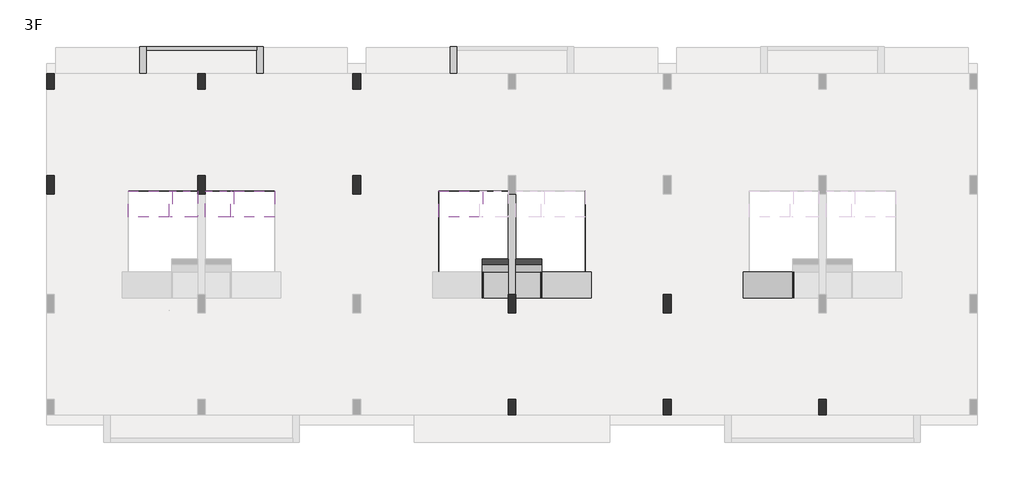
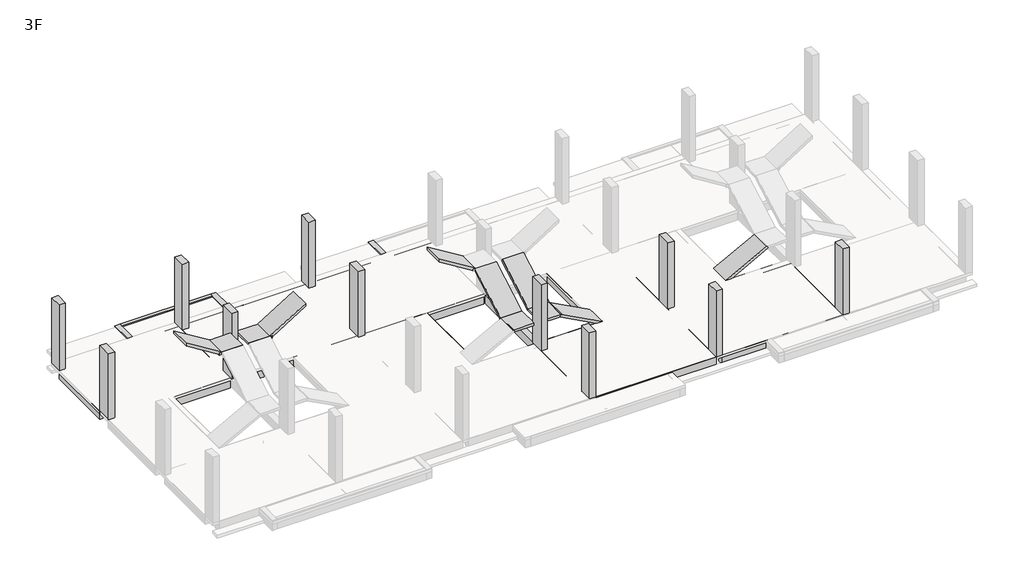
# One storey, part 2 of 3: 36 beams, 11 columns.
"""IFC4 building model written with IfcOpenShell, lengths in millimetres."""

from ifc_helpers import new_model, si_unit, frame, origin, place, context, project, spatial, polyline, outline, extrude, faceted_brep, element, save

model = new_model("IFC4")

# Units and contexts
model_context = context("Model", 3, world=origin())
ifc_project = project(units=[si_unit("LENGTHUNIT", "METRE", prefix="MILLI")], contexts=[model_context])

# Site, building, storey
site = spatial("IfcSite", under=ifc_project)
building = spatial("IfcBuilding", under=site)
storey = spatial("IfcBuildingStorey", under=building, Name="3F", Elevation=7330.0)

# Beams
placement = place(None, origin())
element("IfcBeam", 1, ObjectType="M_Concrete-Rectangular Beam : 1000x120", at=placement, inside=storey, context=model_context, shape_type="Brep", body=[
    faceted_brep([(4600.0000007, 7550.0000002, 9580.0), (4600.0000007, 8550.0000002, 9580.0), (4600.0000007, 8550.0000002, 9460.0), (4600.0000007, 7550.0000002, 9460.0), (5700.0000007, 8550.0000002, 9460.0), (5700.0000007, 8550.0000002, 9580.0), (5700.0000007, 7550.0000002, 9580.0), (5700.0000007, 7609.0063595, 9475.5095719), (5700.0000007, 7581.5414925, 9460.0), (4700.0000007, 7550.0000002, 9580.0), (4700.0000007, 7581.5414925, 9460.0), (4700.0000007, 7550.0000002, 9460.0), (4700.0000007, 7609.0063595, 9475.5095719)], [[[0, 1, 2, 3]], [[4, 5, 6, 7, 8]], [[1, 0, 9, 6, 5]], [[2, 1, 5, 4]], [[3, 2, 4, 8, 10, 11]], [[0, 3, 11, 9]], [[12, 7, 6, 9]], [[7, 12, 10, 8]], [[12, 9, 11, 10]]]),
])
element("IfcBeam", 2, ObjectType="M_Concrete-Rectangular Beam : 1000x120", at=placement, inside=storey, context=model_context, shape_type="Brep", body=[
    faceted_brep([(3019.99996, 7549.9999993, 10630.0), (4715.7503089, 7549.9999993, 9580.0), (4715.7503089, 8549.9999993, 9580.0), (3019.99996, 8549.9999993, 10630.0), (4600.0000007, 8549.9999993, 9580.0), (4600.0000007, 8549.9999993, 9510.5302519), (3020.0, 8549.9999993, 10488.8582245), (4600.0000007, 7549.9999993, 9510.5302519), (3020.0, 7549.9999993, 10488.8582245), (4600.0000007, 7549.9999993, 9580.0), (4700.0000007, 7549.9999993, 9580.0)], [[[0, 1, 2, 3]], [[3, 2, 4, 5, 6]], [[5, 7, 8, 6]], [[1, 0, 8, 7, 9, 10]], [[4, 9, 7, 5]], [[9, 4, 2, 1, 10]], [[0, 3, 6, 8]]]),
])
element("IfcBeam", 3, ObjectType="M_Concrete-Rectangular Beam : 1000x120", at=placement, inside=storey, context=model_context, shape_type="Brep", body=[
    faceted_brep([(7100.0000007, 8550.0000002, 9580.0), (7100.0000007, 7550.0000002, 9580.0), (7100.0000007, 7550.0000002, 9460.0), (7100.0000007, 8550.0000002, 9460.0), (6000.0000007, 8550.0000002, 9580.0), (6000.0000007, 8550.0000002, 9460.0), (6000.0000007, 7581.5414925, 9460.0), (6000.0000007, 7609.0063595, 9475.5095719), (6000.0000007, 7550.0000002, 9580.0), (7000.0000007, 7550.0000002, 9580.0), (7000.0000007, 7550.0000002, 9460.0), (7000.0000007, 7581.5414925, 9460.0), (7000.0000007, 7609.0063595, 9475.5095719)], [[[0, 1, 2, 3]], [[4, 5, 6, 7, 8]], [[1, 0, 4, 8, 9]], [[0, 3, 5, 4]], [[3, 2, 10, 11, 6, 5]], [[2, 1, 9, 10]], [[12, 9, 8, 7]], [[12, 7, 6, 11]], [[9, 12, 11, 10]]]),
])
element("IfcBeam", 4, ObjectType="M_Concrete-Rectangular Beam : 1000x120", at=placement, inside=storey, context=model_context, shape_type="Brep", body=[
    faceted_brep([(6984.2496926, 7549.9999993, 9580.0), (8680.0000414, 7549.9999993, 10630.0), (8680.0, 8549.9999993, 10629.9999744), (6984.2496926, 8549.9999993, 9580.0), (8680.0, 8549.9999993, 10488.8582236), (7100.0000007, 8549.9999993, 9510.5302519), (7100.0000007, 8549.9999993, 9580.0), (7100.0000007, 7549.9999993, 9510.5302519), (8680.0, 7549.9999993, 10488.8582236), (7000.0000007, 7549.9999993, 9580.0), (7100.0000007, 7549.9999993, 9580.0)], [[[0, 1, 2, 3]], [[3, 2, 4, 5, 6]], [[7, 5, 4, 8]], [[1, 0, 9, 10, 7, 8]], [[10, 6, 5, 7]], [[6, 10, 9, 0, 3]], [[2, 1, 8, 4]]]),
])
element("IfcBeam", 5, ObjectType="M_Concrete-Rectangular Beam : 1000x120", at=placement, inside=storey, context=model_context, shape_type="Brep", body=[
    faceted_brep([(16700.0000058, 7550.0000002, 9580.0), (17700.0000058, 7550.0000002, 9580.0), (17700.0000058, 7609.0063595, 9475.5095719), (16700.0000058, 7609.0063595, 9475.5095719), (16700.0000058, 5424.9999998, 8380.0), (16700.0000058, 5484.0063591, 8275.5095719), (17700.0000058, 5484.0063591, 8275.5095719), (17700.0000058, 5424.9999998, 8380.0), (17700.0000058, 5524.9999998, 8298.6589219), (17700.0000058, 7581.5414925, 9460.0), (16700.0000058, 5524.9999998, 8298.6589219), (16700.0000058, 7581.5414925, 9460.0)], [[[0, 1, 2, 3]], [[4, 5, 6, 7]], [[1, 0, 4, 7]], [[2, 1, 7, 6, 8, 9]], [[3, 2, 9, 8, 6, 5, 10, 11]], [[0, 3, 11, 10, 5, 4]]]),
])
element("IfcBeam", 6, ObjectType="M_Concrete-Rectangular Beam : 1000x120", at=placement, inside=storey, context=model_context, shape_type="Brep", body=[
    faceted_brep([(15019.9999651, 7549.9999993, 10630.0), (16715.7503139, 7549.9999993, 9580.0), (16715.7503139, 8549.9999993, 9580.0), (15019.9999651, 8549.9999993, 10630.0), (16600.0000058, 8549.9999993, 9580.0), (16600.0000058, 8549.9999993, 9510.5302519), (15020.0000057, 8549.9999993, 10488.8582241), (16600.0000058, 7549.9999993, 9510.5302519), (15020.0000057, 7549.9999993, 10488.8582241), (16600.0000058, 7549.9999993, 9580.0), (16700.0000058, 7549.9999993, 9580.0)], [[[0, 1, 2, 3]], [[3, 2, 4, 5, 6]], [[5, 7, 8, 6]], [[1, 0, 8, 7, 9, 10]], [[4, 9, 7, 5]], [[9, 4, 2, 1, 10]], [[0, 3, 6, 8]]]),
])
element("IfcBeam", 7, ObjectType="M_Concrete-Rectangular Beam : 1000x120", at=placement, inside=storey, context=model_context, shape_type="Brep", body=[
    faceted_brep([(17700.0000058, 5524.9999998, 8260.0), (16700.0000058, 5524.9999998, 8260.0), (16700.0000058, 5524.9999998, 8298.6589219), (17700.0000058, 5524.9999998, 8298.6589219), (17700.0000058, 4424.9999998, 8260.0), (17700.0000058, 4424.9999998, 8380.0), (16730.4772117, 4424.9999998, 8380.0), (16787.1330628, 4424.9999998, 8274.2166623), (16760.588832, 4424.9999998, 8260.0), (17700.0000058, 5424.9999998, 8380.0), (16700.0000058, 5424.9999998, 8380.0), (16700.0000058, 4424.9999998, 8380.0), (17700.0000058, 5484.0063591, 8275.5095719), (16760.588832, 5424.9999998, 8260.0), (16700.0000058, 5424.9999998, 8260.0), (16700.0000058, 4424.9999998, 8363.6768996), (16700.0000058, 5484.0063591, 8275.5095719), (16700.0000058, 5424.9999998, 8363.6768996), (16730.4772117, 5424.9999998, 8380.0), (16787.1330628, 5424.9999998, 8274.2166623)], [[[0, 1, 2, 3]], [[4, 5, 6, 7, 8]], [[6, 5, 9, 10, 11]], [[5, 4, 0, 3, 12, 9]], [[1, 0, 4, 8, 13, 14]], [[15, 11, 10, 16, 2, 1, 14, 17]], [[6, 18, 19, 7]], [[18, 6, 15, 17]], [[7, 19, 13, 8]], [[19, 18, 17, 14, 13]], [[11, 15, 6]], [[12, 16, 10, 9]], [[16, 12, 3, 2]]]),
])
element("IfcBeam", 8, ObjectType="M_Concrete-Rectangular Beam : 1000x120", at=placement, inside=storey, context=model_context, shape_type="Brep", body=[
    faceted_brep([(18969.5227998, 4424.9999998, 8380.0), (18969.5227998, 5424.9999998, 8380.0), (18912.8669488, 5424.9999998, 8274.2166623), (18912.8669488, 4424.9999998, 8274.2166623), (19000.0000058, 4424.9999998, 8363.6768996), (20930.0000065, 4424.9999998, 7330.0), (20930.0000065, 5424.9999998, 7330.0), (19000.0000058, 5424.9999998, 8363.6768996), (18939.4111796, 4424.9999998, 8260.0), (20675.8338483, 4424.9999998, 7330.0), (18939.4111796, 5424.9999998, 8260.0), (20680.0000058, 5424.9999998, 7327.7686732), (20680.0000058, 4449.9999998, 7327.7686732), (20675.8338483, 4449.9999998, 7330.0), (20680.0000058, 5424.9999998, 7330.0), (20680.0000058, 4449.9999998, 7330.0)], [[[0, 1, 2, 3]], [[1, 0, 4, 5, 6, 7]], [[0, 3, 8, 9, 5, 4]], [[3, 2, 10, 11, 12, 13, 9, 8]], [[2, 1, 7, 6, 14, 11, 10]], [[9, 13, 15, 14, 6, 5]], [[11, 14, 15, 12]], [[15, 13, 12]]]),
])
element("IfcBeam", 9, ObjectType="M_Concrete-Rectangular Beam : 1000x120", at=placement, inside=storey, context=model_context, shape_type="Brep", body=[
    faceted_brep([(19000.0000058, 7550.0000002, 9580.0), (19000.0000058, 7609.0063595, 9475.5095719), (18000.0000058, 7609.0063595, 9475.5095719), (18000.0000058, 7550.0000002, 9580.0), (19000.0000058, 5424.9999998, 8380.0), (18000.0000058, 5424.9999998, 8380.0), (18000.0000058, 5484.0063591, 8275.5095719), (19000.0000058, 5484.0063591, 8275.5095719), (18000.0000058, 7581.5414925, 9460.0), (18000.0000058, 5524.9999998, 8298.6589219), (19000.0000058, 7581.5414925, 9460.0), (19000.0000058, 5524.9999998, 8298.6589219)], [[[0, 1, 2, 3]], [[4, 5, 6, 7]], [[3, 5, 4, 0]], [[2, 8, 9, 6, 5, 3]], [[1, 10, 11, 7, 6, 9, 8, 2]], [[0, 4, 7, 11, 10, 1]]]),
])
element("IfcBeam", 10, ObjectType="M_Concrete-Rectangular Beam : 1000x120", at=placement, inside=storey, context=model_context, shape_type="Brep", body=[
    faceted_brep([(19000.0000058, 5524.9999998, 8260.0), (18000.0000058, 5524.9999998, 8260.0), (18000.0000058, 5524.9999998, 8298.6589219), (19000.0000058, 5524.9999998, 8298.6589219), (18000.0000058, 4424.9999998, 8380.0), (18000.0000058, 4424.9999998, 8260.0), (18939.4111796, 4424.9999998, 8260.0), (18912.8669488, 4424.9999998, 8274.2166623), (18969.5227998, 4424.9999998, 8380.0), (19000.0000058, 4424.9999998, 8380.0), (19000.0000058, 5424.9999998, 8380.0), (18000.0000058, 5424.9999998, 8380.0), (18000.0000058, 5484.0063591, 8275.5095719), (19000.0000058, 5424.9999998, 8260.0), (18939.4111796, 5424.9999998, 8260.0), (19000.0000058, 4424.9999998, 8363.6768996), (19000.0000058, 5424.9999998, 8363.6768996), (19000.0000058, 5484.0063591, 8275.5095719), (18969.5227998, 5424.9999998, 8380.0), (18912.8669488, 5424.9999998, 8274.2166623)], [[[0, 1, 2, 3]], [[4, 5, 6, 7, 8]], [[8, 9, 10, 11, 4]], [[5, 4, 11, 12, 2, 1]], [[1, 0, 13, 14, 6, 5]], [[9, 15, 16, 13, 0, 3, 17, 10]], [[18, 8, 7, 19]], [[8, 18, 16, 15]], [[19, 7, 6, 14]], [[18, 19, 14, 13, 16]], [[15, 9, 8]], [[17, 12, 11, 10]], [[12, 17, 3, 2]]]),
])
element("IfcBeam", 11, ObjectType="M_Concrete-Rectangular Beam : 1000x120", at=placement, inside=storey, context=model_context, shape_type="Brep", body=[
    faceted_brep([(28730.4772098, 5424.9999998, 8380.0), (28730.4772098, 4424.9999998, 8380.0), (28787.1330609, 4424.9999998, 8274.2166623), (28787.1330609, 5424.9999998, 8274.2166623), (28700.0000039, 5424.9999998, 8363.6768996), (26770.0000031, 5424.9999998, 7330.0), (26770.0000031, 4424.9999998, 7330.0), (28700.0000039, 4424.9999998, 8363.6768996), (27024.1661613, 4424.9999998, 7330.0), (28760.5888301, 4424.9999998, 8260.0), (27024.1661613, 4449.9999998, 7330.0), (27020.000004, 4449.9999998, 7327.7686733), (27020.000004, 5424.9999998, 7327.7686733), (28760.5888301, 5424.9999998, 8260.0), (27020.000004, 5424.9999998, 7330.0), (27020.000004, 4449.9999998, 7330.0)], [[[0, 1, 2, 3]], [[1, 0, 4, 5, 6, 7]], [[2, 1, 7, 6, 8, 9]], [[3, 2, 9, 8, 10, 11, 12, 13]], [[0, 3, 13, 12, 14, 5, 4]], [[5, 14, 15, 10, 8, 6]], [[14, 12, 11, 15]], [[10, 15, 11]]]),
])
element("IfcBeam", 12, ObjectType="M_Concrete-Rectangular Beam : 150x500", at=placement, inside=storey, context=model_context, shape_type="SweptSolid", body=[
    extrude(outline(polyline([(7990.0000277, 14150.0000066), (7990.0000277, 14000.0000066), (3709.9999747, 14000.0000066), (3709.9999747, 14150.0000066), (7990.0000277, 14150.0000066)])), frame((0.0, 0.0, 6830.0), z_axis=(0.0, 0.0, 1.0), x_axis=(1.0, 0.0, 0.0)), (0.0, 0.0, 1.0), 500.0),
])
element("IfcBeam", 13, ObjectType="M_Concrete-Rectangular Beam : 250x400", at=placement, inside=storey, context=model_context, shape_type="Brep", body=[
    faceted_brep([(20930.0000058, 8549.9999993, 7330.0), (20680.0000058, 8549.9999993, 7330.0), (20680.0000058, 5424.9999998, 7330.0), (20680.0000058, 4449.9999998, 7330.0), (20930.0000058, 4449.9999998, 7330.0), (20680.0000058, 8549.9999993, 7188.8582241), (20680.0000058, 8549.9999993, 6930.0), (20680.0000058, 4449.9999998, 6930.0), (20680.0000058, 4449.9999998, 7327.7686732), (20930.0000058, 8549.9999993, 6930.0), (20930.0000058, 4449.9999998, 6930.0)], [[[0, 1, 2, 3, 4]], [[1, 5, 6, 7, 8, 3, 2]], [[6, 9, 10, 7]], [[9, 0, 4, 10]], [[1, 0, 9, 6, 5]], [[4, 3, 8, 7, 10]]]),
])
element("IfcBeam", 14, ObjectType="M_Concrete-Rectangular Beam : 250x400", at=placement, inside=storey, context=model_context, shape_type="Brep", body=[
    faceted_brep([(15020.0000057, 8549.9999993, 7330.0), (14770.0000057, 8549.9999993, 7330.0), (14770.0000057, 4449.9999998, 7330.0), (15020.0000057, 4449.9999998, 7330.0), (15020.0000057, 5424.9999998, 7330.0), (15020.0000057, 8549.9999993, 6930.0), (15020.0000057, 8549.9999993, 7188.8582241), (15020.0000057, 4449.9999998, 7327.7686732), (15020.0000057, 4449.9999998, 6930.0), (14770.0000057, 8549.9999993, 6930.0), (14770.0000057, 4449.9999998, 6930.0)], [[[0, 1, 2, 3, 4]], [[5, 6, 0, 4, 3, 7, 8]], [[9, 5, 8, 10]], [[1, 9, 10, 2]], [[1, 0, 6, 5, 9]], [[3, 2, 10, 8, 7]]]),
])
element("IfcBeam", 15, ObjectType="M_Concrete-Rectangular Beam : 250x500", at=placement, inside=storey, context=model_context, shape_type="Brep", body=[
    faceted_brep([(8240.0000277, 14150.0000066, 7330.0), (7990.0000277, 14150.0000066, 7330.0), (7990.0000277, 14000.0000066, 7330.0), (7990.0000277, 13100.0000001, 7330.0), (8240.0000277, 13100.0000001, 7330.0), (7990.0000277, 14150.0000066, 6830.0), (7990.0000277, 14000.0000066, 6830.0), (7990.0000277, 13100.0000001, 6830.0), (8240.0000277, 14150.0000066, 6830.0), (8240.0000277, 13100.0000001, 6830.0)], [[[0, 1, 2, 3, 4]], [[1, 5, 6, 7, 3, 2]], [[5, 8, 9, 7, 6]], [[8, 0, 4, 9]], [[4, 3, 7, 9]], [[1, 0, 8, 5]]]),
])
element("IfcBeam", 16, ObjectType="M_Concrete-Rectangular Beam : 250x500", at=placement, inside=storey, context=model_context, shape_type="Brep", body=[
    faceted_brep([(3709.9999747, 14150.0000066, 7330.0), (3459.9999747, 14150.0000066, 7330.0), (3459.9999747, 13100.0000001, 7330.0), (3709.9999747, 13100.0000001, 7330.0), (3709.9999747, 14000.0000066, 7330.0), (3709.9999747, 14150.0000066, 6830.0), (3709.9999747, 13100.0000001, 6830.0), (3709.9999747, 14000.0000066, 6830.0), (3459.9999747, 14150.0000066, 6830.0), (3459.9999747, 13100.0000001, 6830.0)], [[[0, 1, 2, 3, 4]], [[5, 0, 4, 3, 6, 7]], [[8, 5, 7, 6, 9]], [[1, 8, 9, 2]], [[3, 2, 9, 6]], [[1, 0, 5, 8]]]),
])
element("IfcBeam", 17, ObjectType="M_Concrete-Rectangular Beam : 250x500", at=placement, inside=storey, context=model_context, shape_type="Brep", body=[
    faceted_brep([(15710.0998466, 14150.0000066, 7330.0), (15460.0998466, 14150.0000066, 7330.0), (15460.0998466, 13100.0000001, 7330.0), (15710.0998466, 13100.0000001, 7330.0), (15710.0998466, 14000.0000066, 7330.0), (15710.0998466, 14150.0000066, 6830.0), (15710.0998466, 13100.0000001, 6830.0), (15710.0998466, 14000.0000066, 6830.0), (15460.0998466, 14150.0000066, 6830.0), (15460.0998466, 13100.0000001, 6830.0)], [[[0, 1, 2, 3, 4]], [[5, 0, 4, 3, 6, 7]], [[8, 5, 7, 6, 9]], [[1, 8, 9, 2]], [[3, 2, 9, 6]], [[1, 0, 5, 8]]]),
])
element("IfcBeam", 18, ObjectType="M_Concrete-Rectangular Beam : 300x400", at=placement, inside=storey, context=model_context, shape_type="SweptSolid", body=[
    extrude(outline(polyline([(165.0, 9149.9985388), (-135.0, 9149.9985388), (-135.0, 12500.0000003), (165.0, 12500.0000003), (165.0, 9149.9985388)])), frame((0.0, 0.0, 6930.0), z_axis=(0.0, 0.0, 1.0), x_axis=(1.0, 0.0, 0.0)), (0.0, 0.0, 1.0), 400.0),
])
element("IfcBeam", 19, ObjectType="M_Concrete-Rectangular Beam : 300x400", at=placement, inside=storey, context=model_context, shape_type="SweptSolid", body=[
    extrude(outline(polyline([(18000.0000046, 4550.0000002), (17700.0000046, 4550.0000002), (17700.0000046, 8449.9985388), (18000.0000046, 8449.9985388), (18000.0000046, 4550.0000002)])), frame((0.0, 0.0, 6930.0), z_axis=(0.0, 0.0, 1.0), x_axis=(1.0, 0.0, 0.0)), (0.0, 0.0, 1.0), 400.0),
])
element("IfcBeam", 20, ObjectType="M_Concrete-Rectangular Beam : 300x400", at=placement, inside=storey, context=model_context, shape_type="SweptSolid", body=[
    extrude(outline(polyline([(18000.0000046, 499.9999998), (17700.0000046, 499.9999998), (17700.0000046, 3850.0000002), (18000.0000046, 3850.0000002), (18000.0000046, 499.9999998)])), frame((0.0, 0.0, 6930.0), z_axis=(0.0, 0.0, 1.0), x_axis=(1.0, 0.0, 0.0)), (0.0, 0.0, 1.0), 400.0),
])
element("IfcBeam", 21, ObjectType="M_Concrete-Rectangular Beam : 300x400", at=placement, inside=storey, context=model_context, shape_type="SweptSolid", body=[
    extrude(outline(polyline([(30000.0000031, 499.9999998), (29700.0000031, 499.9999998), (29700.0000031, 3850.0000002), (30000.0000031, 3850.0000002), (30000.0000031, 499.9999998)])), frame((0.0, 0.0, 6930.0), z_axis=(0.0, 0.0, 1.0), x_axis=(1.0, 0.0, 0.0)), (0.0, 0.0, 1.0), 400.0),
])
element("IfcBeam", 22, ObjectType="M_Concrete-Rectangular Beam : 300x400", at=placement, inside=storey, context=model_context, shape_type="SweptSolid", body=[
    extrude(outline(polyline([(24000.000004, 499.9999998), (23700.000004, 499.9999998), (23700.000004, 3850.0000002), (24000.000004, 3850.0000002), (24000.000004, 499.9999998)])), frame((0.0, 0.0, 6930.0), z_axis=(0.0, 0.0, 1.0), x_axis=(1.0, 0.0, 0.0)), (0.0, 0.0, 1.0), 400.0),
])
element("IfcBeam", 23, ObjectType="M_Concrete-Rectangular Beam : 300x400", at=placement, inside=storey, context=model_context, shape_type="SweptSolid", body=[
    extrude(outline(polyline([(24000.000004, 4550.0000002), (23700.000004, 4550.0000002), (23700.000004, 8449.9985388), (24000.000004, 8449.9985388), (24000.000004, 4550.0000002)])), frame((0.0, 0.0, 6930.0), z_axis=(0.0, 0.0, 1.0), x_axis=(1.0, 0.0, 0.0)), (0.0, 0.0, 1.0), 400.0),
])
element("IfcBeam", 24, ObjectType="M_Concrete-Rectangular Beam : 300x400", at=placement, inside=storey, context=model_context, shape_type="SweptSolid", body=[
    extrude(outline(polyline([(6000.0000007, 9149.9985388), (5700.0000007, 9149.9985388), (5700.0000007, 12500.0000003), (6000.0000007, 12500.0000003), (6000.0000007, 9149.9985388)])), frame((0.0, 0.0, 6930.0), z_axis=(0.0, 0.0, 1.0), x_axis=(1.0, 0.0, 0.0)), (0.0, 0.0, 1.0), 400.0),
])
element("IfcBeam", 25, ObjectType="M_Concrete-Rectangular Beam : 300x400", at=placement, inside=storey, context=model_context, shape_type="SweptSolid", body=[
    extrude(outline(polyline([(12000.0000034, 9149.9985388), (11700.0000034, 9149.9985388), (11700.0000034, 12500.0000003), (12000.0000034, 12500.0000003), (12000.0000034, 9149.9985388)])), frame((0.0, 0.0, 6930.0), z_axis=(0.0, 0.0, 1.0), x_axis=(1.0, 0.0, 0.0)), (0.0, 0.0, 1.0), 400.0),
])
element("IfcBeam", 26, ObjectType="M_Concrete-Rectangular Beam : 300x400", at=placement, inside=storey, context=model_context, shape_type="SweptSolid", body=[
    extrude(outline(polyline([(6000.0000007, 13100.0000003), (5700.0000007, 13100.0000001), (5700.0000007, 14000.0000066), (6000.0000007, 14000.0000066), (6000.0000007, 13100.0000003)])), frame((0.0, 0.0, 6880.0), z_axis=(0.0, 0.0, 1.0), x_axis=(1.0, 0.0, 0.0)), (0.0, 0.0, 1.0), 400.0),
])
element("IfcBeam", 27, ObjectType="M_Concrete-Rectangular Beam : 300x500", at=placement, inside=storey, context=model_context, shape_type="Brep", body=[
    faceted_brep([(164.9999993, 13100.0000001, 7330.0), (164.9999993, 12800.0000001, 7330.0), (5700.0000007, 12800.0000001, 7330.0), (5700.0000007, 13100.0000001, 7330.0), (3709.9999747, 13100.0000001, 7330.0), (3459.9999747, 13100.0000001, 7330.0), (164.9999993, 12800.0000001, 6830.0), (5700.0000007, 12800.0000001, 6830.0), (164.9999993, 13100.0000001, 6830.0), (3459.9999747, 13100.0000001, 6830.0), (3709.9999747, 13100.0000001, 6830.0), (5700.0000007, 13100.0000001, 6830.0)], [[[0, 1, 2, 3, 4, 5]], [[1, 6, 7, 2]], [[6, 8, 9, 10, 11, 7]], [[8, 0, 5, 4, 3, 11, 10, 9]], [[1, 0, 8, 6]], [[3, 2, 7, 11]]]),
])
element("IfcBeam", 28, ObjectType="M_Concrete-Rectangular Beam : 300x500", at=placement, inside=storey, context=model_context, shape_type="Brep", body=[
    faceted_brep([(165.0, 8849.9999993, 7330.0), (165.0, 8549.9999993, 7330.0), (2770.0, 8549.9999993, 7330.0), (3020.0, 8549.9999993, 7330.0), (5700.0000007, 8549.9999993, 7330.0), (5700.0000007, 8849.9999993, 7330.0), (165.0, 8549.9999993, 6830.0), (5700.0000007, 8549.9999993, 6830.0), (165.0, 8849.9999993, 6830.0), (5700.0000007, 8849.9999993, 6830.0)], [[[0, 1, 2, 3, 4, 5]], [[1, 6, 7, 4, 3, 2]], [[6, 8, 9, 7]], [[8, 0, 5, 9]], [[1, 0, 8, 6]], [[5, 4, 7, 9]]]),
])
element("IfcBeam", 29, ObjectType="M_Concrete-Rectangular Beam : 300x500", at=placement, inside=storey, context=model_context, shape_type="Brep", body=[
    faceted_brep([(6000.0000007, 13100.0000001, 7330.0), (6000.0000007, 12800.0000001, 7330.0), (11700.0000034, 12800.0000001, 7330.0), (11700.0000034, 13100.0000001, 7330.0), (8240.0000277, 13100.0000001, 7330.0), (7990.0000277, 13100.0000001, 7330.0), (6000.0000007, 12800.0000001, 6830.0), (11700.0000034, 12800.0000001, 6830.0), (6000.0000007, 13100.0000001, 6830.0), (7990.0000277, 13100.0000001, 6830.0), (8240.0000277, 13100.0000001, 6830.0), (11700.0000034, 13100.0000001, 6830.0)], [[[0, 1, 2, 3, 4, 5]], [[1, 6, 7, 2]], [[6, 8, 9, 10, 11, 7]], [[8, 0, 5, 4, 3, 11, 10, 9]], [[1, 0, 8, 6]], [[3, 2, 7, 11]]]),
])
element("IfcBeam", 30, ObjectType="M_Concrete-Rectangular Beam : 300x500", at=placement, inside=storey, context=model_context, shape_type="Brep", body=[
    faceted_brep([(6000.0000007, 8849.9999993, 7330.0), (6000.0, 8549.9999993, 7330.0), (8680.0, 8549.9999993, 7330.0), (8930.0, 8549.9999993, 7330.0), (11700.0000034, 8549.9999993, 7330.0), (11700.0000034, 8849.9999993, 7330.0), (6000.0000007, 8549.9999993, 6830.0), (11700.0000034, 8549.9999993, 6830.0), (6000.0000007, 8849.9999993, 6830.0), (11700.0000034, 8849.9999993, 6830.0)], [[[0, 1, 2, 3, 4, 5]], [[1, 6, 7, 4, 3, 2]], [[6, 8, 9, 7]], [[8, 0, 5, 9]], [[8, 6, 1, 0]], [[5, 4, 7, 9]]]),
])
element("IfcBeam", 31, ObjectType="M_Concrete-Rectangular Beam : 300x500", at=placement, inside=storey, context=model_context, shape_type="Brep", body=[
    faceted_brep([(12000.0000034, 13100.0000001, 7330.0), (12000.0000034, 12800.0000001, 7330.0), (17700.0000058, 12800.0000001, 7330.0), (17700.0000058, 13100.0000001, 7330.0), (15710.0998466, 13100.0000001, 7330.0), (15460.0998466, 13100.0000001, 7330.0), (12000.0000034, 12800.0000001, 6830.0), (17700.0000058, 12800.0000001, 6830.0), (12000.0000034, 13100.0000001, 6830.0), (15460.0998466, 13100.0000001, 6830.0), (15710.0998466, 13100.0000001, 6830.0), (17700.0000058, 13100.0000001, 6830.0)], [[[0, 1, 2, 3, 4, 5]], [[1, 6, 7, 2]], [[6, 8, 9, 10, 11, 7]], [[8, 0, 5, 4, 3, 11, 10, 9]], [[8, 6, 1, 0]], [[3, 2, 7, 11]]]),
])
element("IfcBeam", 32, ObjectType="M_Concrete-Rectangular Beam : 300x500", at=placement, inside=storey, context=model_context, shape_type="Brep", body=[
    faceted_brep([(12000.0000034, 8849.9999993, 7330.0), (12000.0000027, 8549.9999993, 7330.0), (14770.0000057, 8549.9999993, 7330.0), (15020.0000057, 8549.9999993, 7330.0), (17700.0000058, 8549.9999993, 7330.0), (17700.0000058, 8849.9999993, 7330.0), (12000.0000034, 8549.9999993, 6830.0), (17700.0000058, 8549.9999993, 6830.0), (12000.0000034, 8849.9999993, 6830.0), (17700.0000058, 8849.9999993, 6830.0)], [[[0, 1, 2, 3, 4, 5]], [[1, 6, 7, 4, 3, 2]], [[6, 8, 9, 7]], [[8, 0, 5, 9]], [[8, 6, 1, 0]], [[5, 4, 7, 9]]]),
])
element("IfcBeam", 33, ObjectType="M_Concrete-Rectangular Beam : 300x500", at=placement, inside=storey, context=model_context, shape_type="Brep", body=[
    faceted_brep([(18000.0000058, 4449.9999998, 7330.0), (18000.0000058, 4149.9999998, 7330.0), (23700.0000047, 4149.9999998, 7330.0), (23700.0000047, 4449.9999998, 7330.0), (20930.0000058, 4449.9999998, 7330.0), (20680.0000058, 4449.9999998, 7330.0), (20675.8338483, 4449.9999998, 7330.0), (18000.0000058, 4149.9999998, 6830.0), (23700.0000047, 4149.9999998, 6830.0), (18000.0000058, 4449.9999998, 6830.0), (23700.0000047, 4449.9999998, 6830.0)], [[[0, 1, 2, 3, 4, 5, 6]], [[1, 7, 8, 2]], [[7, 9, 10, 8]], [[9, 0, 6, 5, 4, 3, 10]], [[1, 0, 9, 7]], [[3, 2, 8, 10]]]),
])
element("IfcBeam", 34, ObjectType="M_Concrete-Rectangular Beam : 300x500", at=placement, inside=storey, context=model_context, shape_type="Brep", body=[
    faceted_brep([(18000.0000058, 199.9999993, 7330.0), (18000.0000058, -100.0000007, 7330.0), (23700.0000047, -100.0000007, 7330.0), (23700.0000047, 199.9999993, 7330.0), (18000.0000058, -100.0000007, 6830.0), (21380.0998336, -100.0000007, 6830.0), (21630.0998336, -100.0000007, 6830.0), (23700.0000047, -100.0000007, 6830.0), (18000.0000058, 199.9999993, 6830.0), (23700.0000047, 199.9999993, 6830.0)], [[[0, 1, 2, 3]], [[1, 4, 5, 6, 7, 2]], [[4, 8, 9, 7, 6, 5]], [[8, 0, 3, 9]], [[1, 0, 8, 4]], [[3, 2, 7, 9]]]),
])
element("IfcBeam", 35, ObjectType="M_Concrete-Rectangular Beam : 300x500", at=placement, inside=storey, context=model_context, shape_type="Brep", body=[
    faceted_brep([(24000.0000047, 4449.9999998, 7330.0), (24000.000004, 4149.9999998, 7330.0), (29700.0000039, 4149.9999998, 7330.0), (29700.0000039, 4449.9999998, 7330.0), (27024.1661613, 4449.9999998, 7330.0), (27020.000004, 4449.9999998, 7330.0), (26770.000004, 4449.9999998, 7330.0), (24000.0000047, 4149.9999998, 6830.0), (29700.0000039, 4149.9999998, 6830.0), (24000.0000047, 4449.9999998, 6830.0), (29700.0000039, 4449.9999998, 6830.0)], [[[0, 1, 2, 3, 4, 5, 6]], [[1, 7, 8, 2]], [[7, 9, 10, 8]], [[9, 0, 6, 5, 4, 3, 10]], [[9, 7, 1, 0]], [[3, 2, 8, 10]]]),
])
element("IfcBeam", 36, ObjectType="M_Concrete-Rectangular Beam : 300x500", at=placement, inside=storey, context=model_context, shape_type="Brep", body=[
    faceted_brep([(24000.000004, 202.2719854, 7330.0), (24000.0000047, -97.7280146, 7330.0), (26070.012858, -97.7280146, 7330.0), (26320.012858, -97.7280146, 7330.0), (29700.0000039, -97.7280146, 7330.0), (29700.0000039, 202.2719854, 7330.0), (24000.0000047, -97.7280146, 6830.0), (26070.012858, -97.7280146, 6830.0), (26320.012858, -97.7280146, 6830.0), (29700.0000039, -97.7280146, 6830.0), (24000.0000047, 202.2719854, 6830.0), (29700.0000039, 202.2719854, 6830.0)], [[[0, 1, 2, 3, 4, 5]], [[1, 6, 7, 8, 9, 4, 3, 2]], [[6, 10, 11, 9, 8, 7]], [[10, 0, 5, 11]], [[6, 1, 0, 10]], [[5, 4, 9, 11]]]),
])

# Columns
element("IfcColumn", 37, ObjectType="M_Concrete-Rectangular-Column : 300x600", at=placement, inside=storey, context=model_context, shape_type="SweptSolid", body=[
    extrude(outline(polyline([(164.9999993, 13100.0000005), (164.9999993, 12500.0000005), (-135.0000007, 12500.0000005), (-135.0000007, 13100.0000005), (164.9999993, 13100.0000005)])), frame((0.0, 0.0, 7330.0), z_axis=(0.0, 0.0, 1.0), x_axis=(1.0, 0.0, 0.0)), (0.0, 0.0, 1.0), 3300.0),
])
element("IfcColumn", 38, ObjectType="M_Concrete-Rectangular-Column : 300x600", at=placement, inside=storey, context=model_context, shape_type="SweptSolid", body=[
    extrude(outline(polyline([(18000.0000058, 500.0), (18000.0000058, -100.0), (17700.0000058, -100.0), (17700.0000058, 500.0), (18000.0000058, 500.0)])), frame((0.0, 0.0, 7330.0), z_axis=(0.0, 0.0, 1.0), x_axis=(1.0, 0.0, 0.0)), (0.0, 0.0, 1.0), 3300.0),
])
element("IfcColumn", 39, ObjectType="M_Concrete-Rectangular-Column : 300x600", at=placement, inside=storey, context=model_context, shape_type="SweptSolid", body=[
    extrude(outline(polyline([(24000.0000047, 500.0), (24000.0000047, -100.0), (23700.0000047, -100.0), (23700.0000047, 500.0), (24000.0000047, 500.0)])), frame((0.0, 0.0, 7330.0), z_axis=(0.0, 0.0, 1.0), x_axis=(1.0, 0.0, 0.0)), (0.0, 0.0, 1.0), 3300.0),
])
element("IfcColumn", 40, ObjectType="M_Concrete-Rectangular-Column : 300x600", at=placement, inside=storey, context=model_context, shape_type="SweptSolid", body=[
    extrude(outline(polyline([(6000.0000007, 13100.0000005), (6000.0000007, 12500.0000005), (5700.0000007, 12500.0000005), (5700.0000007, 13100.0000005), (6000.0000007, 13100.0000005)])), frame((0.0, 0.0, 7330.0), z_axis=(0.0, 0.0, 1.0), x_axis=(1.0, 0.0, 0.0)), (0.0, 0.0, 1.0), 3300.0),
])
element("IfcColumn", 41, ObjectType="M_Concrete-Rectangular-Column : 300x600", at=placement, inside=storey, context=model_context, shape_type="SweptSolid", body=[
    extrude(outline(polyline([(12000.0000034, 13100.0000005), (12000.0000034, 12500.0000005), (11700.0000034, 12500.0000005), (11700.0000034, 13100.0000005), (12000.0000034, 13100.0000005)])), frame((0.0, 0.0, 7330.0), z_axis=(0.0, 0.0, 1.0), x_axis=(1.0, 0.0, 0.0)), (0.0, 0.0, 1.0), 3300.0),
])
element("IfcColumn", 42, ObjectType="M_Concrete-Rectangular-Column : 300x600", at=placement, inside=storey, context=model_context, shape_type="SweptSolid", body=[
    extrude(outline(polyline([(30000.0000039, 500.0), (30000.0000039, -100.0), (29700.0000039, -100.0), (29700.0000039, 500.0), (30000.0000039, 500.0)])), frame((0.0, 0.0, 7330.0), z_axis=(0.0, 0.0, 1.0), x_axis=(1.0, 0.0, 0.0)), (0.0, 0.0, 1.0), 3300.0),
])
element("IfcColumn", 43, ObjectType="M_Concrete-Rectangular-Column : 300x700", at=placement, inside=storey, context=model_context, shape_type="SweptSolid", body=[
    extrude(outline(polyline([(164.9649925, 9150.0000002), (164.9649925, 8450.0000002), (-135.0350075, 8450.0000002), (-135.0350075, 9150.0000002), (164.9649925, 9150.0000002)])), frame((0.0, 0.0, 7330.0), z_axis=(0.0, 0.0, 1.0), x_axis=(1.0, 0.0, 0.0)), (0.0, 0.0, 1.0), 3300.0),
])
element("IfcColumn", 44, ObjectType="M_Concrete-Rectangular-Column : 300x700", at=placement, inside=storey, context=model_context, shape_type="SweptSolid", body=[
    extrude(outline(polyline([(18000.0000058, 4550.0000002), (18000.0000058, 3850.0000002), (17700.0000058, 3850.0000002), (17700.0000058, 4550.0000002), (18000.0000058, 4550.0000002)])), frame((0.0, 0.0, 7330.0), z_axis=(0.0, 0.0, 1.0), x_axis=(1.0, 0.0, 0.0)), (0.0, 0.0, 1.0), 3300.0),
])
element("IfcColumn", 45, ObjectType="M_Concrete-Rectangular-Column : 300x700", at=placement, inside=storey, context=model_context, shape_type="SweptSolid", body=[
    extrude(outline(polyline([(24000.0000047, 4550.0000002), (24000.0000047, 3850.0000002), (23700.0000047, 3850.0000002), (23700.0000047, 4550.0000002), (24000.0000047, 4550.0000002)])), frame((0.0, 0.0, 7330.0), z_axis=(0.0, 0.0, 1.0), x_axis=(1.0, 0.0, 0.0)), (0.0, 0.0, 1.0), 3300.0),
])
element("IfcColumn", 46, ObjectType="M_Concrete-Rectangular-Column : 300x700", at=placement, inside=storey, context=model_context, shape_type="SweptSolid", body=[
    extrude(outline(polyline([(5999.9649933, 9150.0000002), (5999.9649933, 8450.0000002), (5699.9649933, 8450.0000002), (5699.9649933, 9150.0000002), (5999.9649933, 9150.0000002)])), frame((0.0, 0.0, 7330.0), z_axis=(0.0, 0.0, 1.0), x_axis=(1.0, 0.0, 0.0)), (0.0, 0.0, 1.0), 3300.0),
])
element("IfcColumn", 47, ObjectType="M_Concrete-Rectangular-Column : 300x700", at=placement, inside=storey, context=model_context, shape_type="SweptSolid", body=[
    extrude(outline(polyline([(11999.964996, 9150.0000002), (11999.964996, 8450.0000002), (11699.964996, 8450.0000002), (11699.964996, 9150.0000002), (11999.964996, 9150.0000002)])), frame((0.0, 0.0, 7330.0), z_axis=(0.0, 0.0, 1.0), x_axis=(1.0, 0.0, 0.0)), (0.0, 0.0, 1.0), 3300.0),
])

save(model, "model.ifc")

# Revit data of these elements
# Type "M_Concrete-Rectangular Beam : 1000x120"
#   Length [instance default] = 1524 mm
#   b = 1000 mm
#   h = 120 mm
#   Structural Material [instance default] = Concrete, Cast-in-Place gray
#   Assembly Code = ""
# Type "M_Concrete-Rectangular Beam : 150x500"
#   Length [instance default] = 1524 mm
#   b = 150 mm
#   h = 500 mm
#   Structural Material [instance default] = Concrete, Cast-in-Place gray
#   Assembly Code = ""
# Type "M_Concrete-Rectangular Beam : 250x400"
#   Length [instance default] = 1524 mm
#   b = 250 mm
#   h = 400 mm
#   Structural Material [instance default] = Concrete, Cast-in-Place gray
#   Assembly Code = ""
# Type "M_Concrete-Rectangular Beam : 250x500"
#   Length [instance default] = 1524 mm
#   b = 250 mm
#   h = 500 mm
#   Structural Material [instance default] = Concrete, Cast-in-Place gray
#   Assembly Code = ""
# Type "M_Concrete-Rectangular Beam : 300x400"
#   Length [instance default] = 1524 mm
#   b = 300 mm
#   h = 400 mm
#   Structural Material [instance default] = Concrete, Cast-in-Place gray
#   Assembly Code = ""
# Type "M_Concrete-Rectangular Beam : 300x500"
#   Length [instance default] = 1524 mm
#   b = 300 mm
#   h = 500 mm
#   Structural Material [instance default] = Concrete, Cast-in-Place gray
#   Assembly Code = ""
# Type "M_Concrete-Rectangular-Column : 300x600"
#   b = 300 mm
#   h = 600 mm
#   Structural Material [instance default] = Concrete, Cast-in-Place gray
# Type "M_Concrete-Rectangular-Column : 300x700"
#   b = 300 mm
#   h = 700 mm
#   Structural Material [instance default] = Concrete, Cast-in-Place gray
# Elements 1, 2, 3, 4, 5, 6, 7, 9, 10 (IfcBeam, "M_Concrete-Rectangular Beam : 1000x120")
#   COF_GEN__Name = "STAIR"
#   Structural Material = Concrete, Cast-in-Place gray
#   Phase Created = New Construction
#   Materials on its faces: "Concrete, Cast-in-Place gray"
# Elements 8, 11 (IfcBeam, "M_Concrete-Rectangular Beam : 1000x120")
#   Comments = ""
#   COF_GEN__Name = "STAIR"
#   Structural Material = Concrete, Cast-in-Place gray
#   Phase Created = New Construction
#   Materials on its faces: "Concrete, Cast-in-Place gray"
# Element 12 (IfcBeam, "M_Concrete-Rectangular Beam : 150x500")
#   Comments = ""
#   COF_CON__WorkItemNumber = "SH3-A-03F"
#   COF_GEN__Name = "DP3"
#   Phase Created = New Construction
#   Materials on its faces: "Concrete, Cast-in-Place gray"
# Elements 13, 14 (IfcBeam, "M_Concrete-Rectangular Beam : 250x400")
#   Comments = ""
#   COF_CON__WorkItemNumber = "SH3-A-03F"
#   COF_GEN__Name = "DP1"
#   Structural Material = Concrete, Cast-in-Place gray
#   Phase Created = New Construction
#   Materials on its faces: "Concrete, Cast-in-Place gray"
# Elements 15, 16, 17 (IfcBeam, "M_Concrete-Rectangular Beam : 250x500")
#   Comments = ""
#   COF_GEN__Name = "DP2"
#   Structural Material = Concrete, Cast-in-Place gray
#   Phase Created = New Construction
#   Materials on its faces: "Concrete, Cast-in-Place gray"
# Elements 18, 22, 23, 25 (IfcBeam, "M_Concrete-Rectangular Beam : 300x400")
#   Comments = ""
#   COF_CON__WorkItemNumber = "SH3-A-03F"
#   COF_GEN__Name = "D3"
#   Structural Material = Concrete, Cast-in-Place gray
#   Phase Created = New Construction
#   Materials on its faces: "Concrete, Cast-in-Place gray"
# Elements 19, 20, 21, 24, 26 (IfcBeam, "M_Concrete-Rectangular Beam : 300x400")
#   Comments = ""
#   COF_CON__WorkItemNumber = "SH3-A-03F"
#   COF_GEN__Name = "D5"
#   Structural Material = Concrete, Cast-in-Place gray
#   Phase Created = New Construction
#   Materials on its faces: "Concrete, Cast-in-Place gray"
# Elements 27, 29, 31, 34, 36 (IfcBeam, "M_Concrete-Rectangular Beam : 300x500")
#   Comments = ""
#   COF_CON__WorkItemNumber = "SH3-A-03F"
#   COF_GEN__Name = "D1"
#   Structural Material = Concrete, Cast-in-Place gray
#   Phase Created = New Construction
#   Materials on its faces: "Concrete, Cast-in-Place gray"
# Elements 28, 30, 32, 33, 35 (IfcBeam, "M_Concrete-Rectangular Beam : 300x500")
#   Comments = ""
#   COF_CON__WorkItemNumber = "SH3-A-03F"
#   COF_GEN__Name = "D2"
#   Structural Material = Concrete, Cast-in-Place gray
#   Phase Created = New Construction
#   Materials on its faces: "Concrete, Cast-in-Place gray"
# Elements 37, 39, 40, 41, 42 (IfcColumn, "M_Concrete-Rectangular-Column : 300x600")
#   Comments = ""
#   COF_CON__WorkItemNumber = "SH3-A-04F"
#   COF_GEN__Name = "C1"
#   Structural Material = Concrete, Cast-in-Place gray
#   Phase Created = New Construction
#   Materials on its faces: "Concrete, Cast-in-Place gray"
# Element 38 (IfcColumn, "M_Concrete-Rectangular-Column : 300x600")
#   Comments = ""
#   COF_CON__WorkItemNumber = "SH3-A-04F"
#   COF_GEN__Name = "C2"
#   Structural Material = Concrete, Cast-in-Place gray
#   Phase Created = New Construction
#   Materials on its faces: "Concrete, Cast-in-Place gray"
# Element 43 (IfcColumn, "M_Concrete-Rectangular-Column : 300x700")
#   Comments = ""
#   COF_CON__WorkItemNumber = "SH3-A-04F"
#   COF_GEN__Name = "C3"
#   Structural Material = Concrete, Cast-in-Place gray
#   Phase Created = New Construction
#   Materials on its faces: "Concrete, Cast-in-Place gray"
# Element 44 (IfcColumn, "M_Concrete-Rectangular-Column : 300x700")
#   Comments = ""
#   COF_CON__WorkItemNumber = "SH3-A-04F"
#   COF_GEN__Name = "C6"
#   Structural Material = Concrete, Cast-in-Place gray
#   Phase Created = New Construction
#   Materials on its faces: "Concrete, Cast-in-Place gray"
# Elements 45, 47 (IfcColumn, "M_Concrete-Rectangular-Column : 300x700")
#   Comments = ""
#   COF_CON__WorkItemNumber = "SH3-A-04F"
#   COF_GEN__Name = "C5"
#   Structural Material = Concrete, Cast-in-Place gray
#   Phase Created = New Construction
#   Materials on its faces: "Concrete, Cast-in-Place gray"
# Element 46 (IfcColumn, "M_Concrete-Rectangular-Column : 300x700")
#   Comments = ""
#   COF_CON__WorkItemNumber = "SH3-A-04F"
#   COF_GEN__Name = "C4"
#   Structural Material = Concrete, Cast-in-Place gray
#   Phase Created = New Construction
#   Materials on its faces: "Concrete, Cast-in-Place gray"
# Materials
#   "Concrete, Cast-in-Place gray": class "Concrete", colour RGB 207 208 204, transparency 0, Description = "Cast-in-place concrete", Cost = 0
